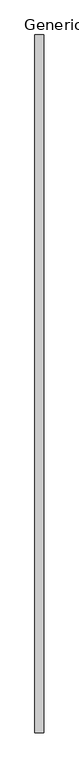
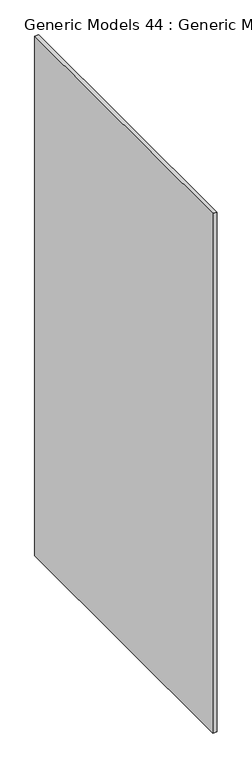
"""IFC4 building model written with IfcOpenShell, lengths in millimetres: proxy geometry, Generic Models 44 : Generic Models 1."""

from ifc_helpers import new_model, si_unit, frame, origin, place, context, project, spatial, polyline, outline, extrude, source, transform, mapped, element, save


def generic_models_44_generic_models_1_ce885a63(model_context):
    return source(origin(), model_context, "Body", "SweptSolid", [
        extrude(outline(polyline([(51019.075, 1219.2), (51019.075, 0.0), (51003.2, 0.0), (51003.2, 1219.2), (51019.075, 1219.2)])), frame((0.0, 0.0, 3054.35), z_axis=(0.0, 0.0, 1.0), x_axis=(1.0, 0.0, 0.0)), (0.0, 0.0, 1.0), 2168.128125),
    ])


if __name__ == "__main__":
    model = new_model("IFC4")
    model_context = context("Model", 3, world=origin())
    ifc_project = project(units=[si_unit("LENGTHUNIT", "METRE", prefix="MILLI")], contexts=[model_context])
    site = spatial("IfcSite", under=ifc_project)
    building = spatial("IfcBuilding", under=site)
    placement = place(None, origin())
    generic_models_44_generic_models_1_shape = generic_models_44_generic_models_1_ce885a63(model_context)
    element("IfcBuildingElementProxy", 1, Name="Generic Models 44 : Generic Models 1", ObjectType="Generic Models 44 : Generic Models 1", at=placement, inside=building, context=model_context, shape_type="MappedRepresentation", body=[
        mapped(generic_models_44_generic_models_1_shape, transform((0.0, 0.0, 0.0), x_axis=(1.0, 0.0, 0.0), y_axis=(0.0, 1.0, 0.0), z_axis=(0.0, 0.0, 1.0))),
    ])
    save(model, "model.ifc")

# Revit data of these elements
# Element 1 (IfcBuildingElementProxy, "Generic Models 44 : Generic Models 1")
#   Materials on its faces: "5/8\" GYP. BD"
# Materials
#   "5/8\" GYP. BD": class "Generic", colour RGB 255 255 255, transparency 0, Description = "Gypsum Wall Board", Cost = 0
